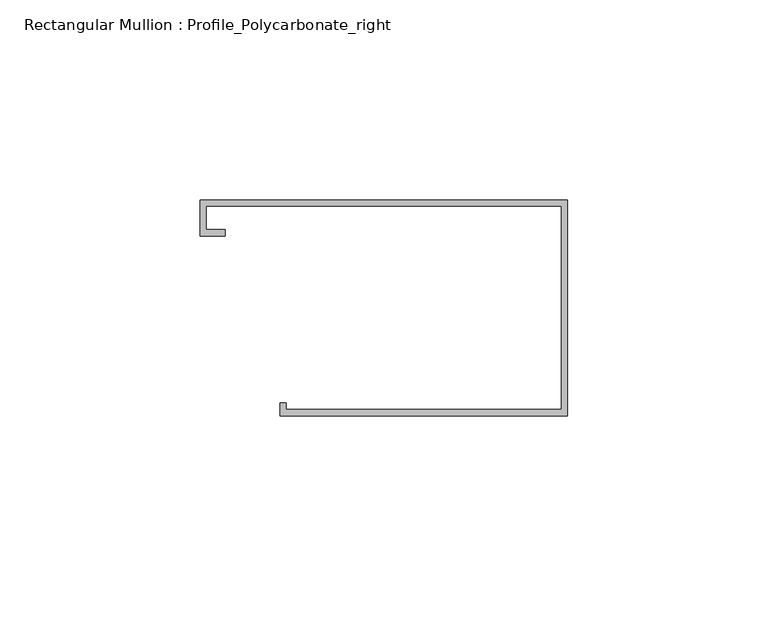
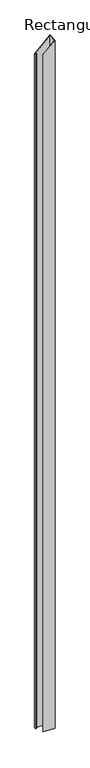
"""IFC4 building model written with IfcOpenShell, lengths in millimetres: member geometry, Rectangular Mullion : Profile_Polycarbonate_right."""

from ifc_helpers import new_model, si_unit, origin, place, context, project, spatial, faceted_brep, source, transform, mapped, element, save


def rectangular_mullion_profile_polycarbonate_right_e985b2b6(model_context):
    return source(origin(), model_context, "Body", "Brep", [
        faceted_brep([(0.0, 28.984575, -4369.9243931), (0.0, -25.015825, -4369.9243931), (-71.9836, -25.015825, -4369.9243931), (-71.9836, -21.840825, -4369.9243931), (-70.3961, -21.840825, -4369.9243931), (-70.3961, -23.428325, -4369.9243931), (-1.5875, -23.428325, -4369.9243931), (-1.5875, 27.397075, -4369.9243931), (-90.4113, 27.397075, -4369.9243931), (-90.4113, 21.580475, -4369.9243931), (-85.6488, 21.580475, -4369.9243931), (-85.6488, 19.992975, -4369.9243931), (-91.9988, 19.992975, -4369.9243931), (-91.9988, 28.984575, -4369.9243931), (-91.9988, 28.984575, -88.2453421), (0.0, 28.984575, 0.0), (-91.9988, 19.992975, -88.2453421), (-85.6488, 19.992975, -82.1544157), (-85.6488, 21.580475, -82.1544157), (-90.4113, 21.580475, -86.7226105), (-90.4113, 27.397075, -86.7226105), (-1.5875, 27.397075, -1.5227316), (-1.5875, -23.428325, -1.5227316), (-70.3961, -23.428325, -67.5240104), (-70.3961, -21.840825, -67.5240104), (-71.9836, -21.840825, -69.046742), (-71.9836, -25.015825, -69.046742), (0.0, -25.015825, 0.0)], [[[0, 1, 2, 3, 4, 5, 6, 7, 8, 9, 10, 11, 12, 13]], [[14, 15, 0, 13]], [[16, 14, 13, 12]], [[17, 16, 12, 11]], [[18, 17, 11, 10]], [[19, 18, 10, 9]], [[20, 19, 9, 8]], [[21, 20, 8, 7]], [[22, 21, 7, 6]], [[23, 22, 6, 5]], [[24, 23, 5, 4]], [[25, 24, 4, 3]], [[26, 25, 3, 2]], [[27, 26, 2, 1]], [[15, 27, 1, 0]], [[15, 14, 16, 17, 18, 19, 20, 21, 22, 23, 24, 25, 26, 27]]]),
    ])


if __name__ == "__main__":
    model = new_model("IFC4")
    model_context = context("Model", 3, world=origin())
    ifc_project = project(units=[si_unit("LENGTHUNIT", "METRE", prefix="MILLI")], contexts=[model_context])
    site = spatial("IfcSite", under=ifc_project)
    building = spatial("IfcBuilding", under=site)
    placement = place(None, origin())
    rectangular_mullion_profile_polycarbonate_right_shape = rectangular_mullion_profile_polycarbonate_right_e985b2b6(model_context)
    element("IfcMember", 1, ObjectType="Rectangular Mullion : Profile_Polycarbonate_right", at=placement, inside=building, context=model_context, shape_type="MappedRepresentation", body=[
        mapped(rectangular_mullion_profile_polycarbonate_right_shape, transform((0.0, 0.0, 0.0), x_axis=(1.0, 0.0, 0.0), y_axis=(0.0, 1.0, 0.0), z_axis=(0.0, 0.0, 1.0))),
    ])
    save(model, "model.ifc")

# Revit data of these elements
# Type "Rectangular Mullion : Profile_Polycarbonate_right"
#   built-in parameter 1007322 = 0.177167 (stored number, unit not read)
#   built-in parameter 1007321 = 0 (stored number, unit not read)
#   built-in parameter 1007320 = 0.00520833 (stored number, unit not read)
